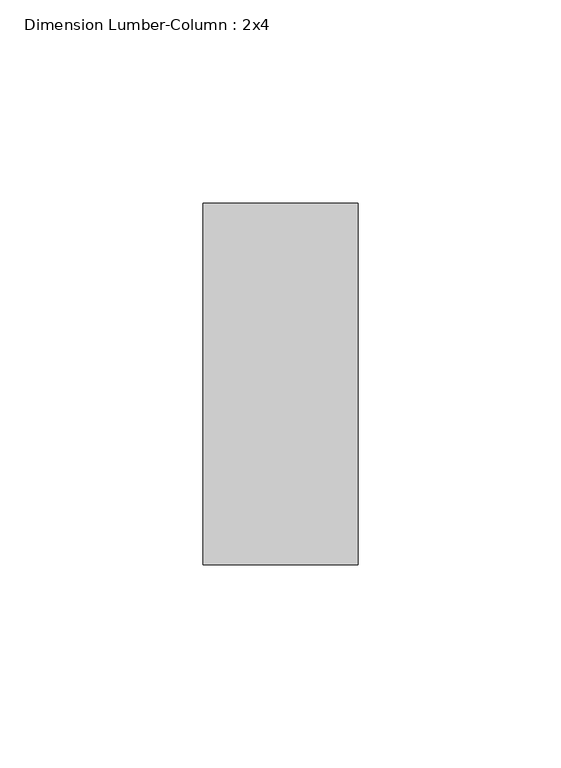
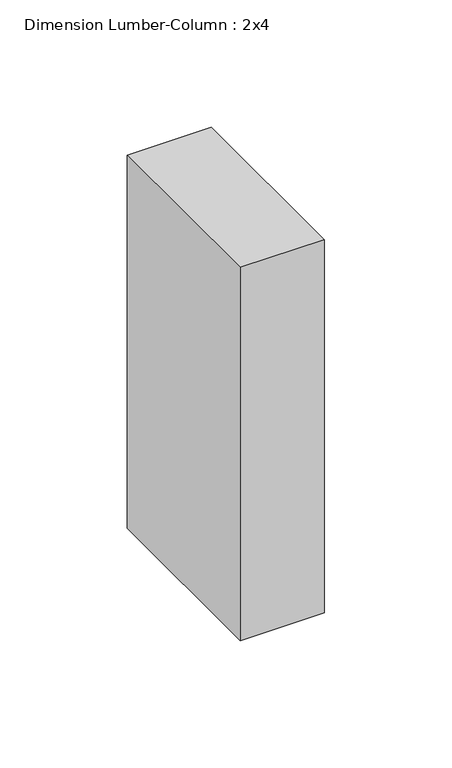
"""IFC4 building model written with IfcOpenShell, lengths in millimetres: column geometry, Dimension Lumber-Column : 2x4."""

from ifc_helpers import new_model, si_unit, frame, origin, place, context, project, spatial, polyline, outline, extrude, source, transform, mapped, element, save


def dimension_lumber_column_2x4_ba6c0a06(model_context):
    return source(origin(), model_context, "Body", "SweptSolid", [
        extrude(outline(polyline([(19.05, -44.45), (-19.05, -44.45), (-19.05, 44.45), (19.05, 44.45), (19.05, -44.45)])), frame((0.0, 0.0, 2208.609375), z_axis=(0.0, 0.0, 1.0), x_axis=(1.0, 0.0, 0.0)), (0.0, 0.0, 1.0), 178.990625),
    ])


if __name__ == "__main__":
    model = new_model("IFC4")
    model_context = context("Model", 3, world=origin())
    ifc_project = project(units=[si_unit("LENGTHUNIT", "METRE", prefix="MILLI")], contexts=[model_context])
    site = spatial("IfcSite", under=ifc_project)
    building = spatial("IfcBuilding", under=site)
    placement = place(None, origin())
    dimension_lumber_column_2x4_shape = dimension_lumber_column_2x4_ba6c0a06(model_context)
    element("IfcColumn", 1, ObjectType="Dimension Lumber-Column : 2x4", at=placement, inside=building, context=model_context, shape_type="MappedRepresentation", body=[
        mapped(dimension_lumber_column_2x4_shape, transform((0.0, 0.0, 0.0), x_axis=(1.0, 0.0, 0.0), y_axis=(0.0, 1.0, 0.0), z_axis=(0.0, 0.0, 1.0))),
    ])
    save(model, "model.ifc")

# Revit data of these elements
# Type "Dimension Lumber-Column : 2x4"
#   Int Type = "Interior"
#   Assembly Code = "B10"
#   Cost = 8.05
#   A = 0.0364583 SF
#   b = 0' - 1 1/2"
#   d = 0' - 3 1/2"
#   Structural Material [instance default] = Softwood, Lumber
# Element 1 (IfcColumn, "Dimension Lumber-Column : 2x4")
#   Structural Material = Douglas Fir #2
#   Materials on its faces: "Douglas Fir #2"
# Materials
#   "Softwood, Lumber": class "Wood", colour RGB 223 192 134, transparency 0, Description = "Pinus Echinata", Cost = 0
#   "Douglas Fir #2": class "Wood", colour RGB 223 192 134, transparency 0, Description = "Pinus Echinata", Cost = 0
